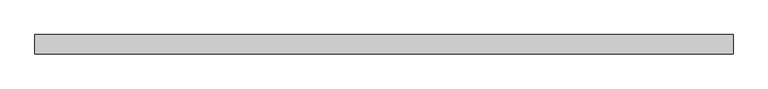
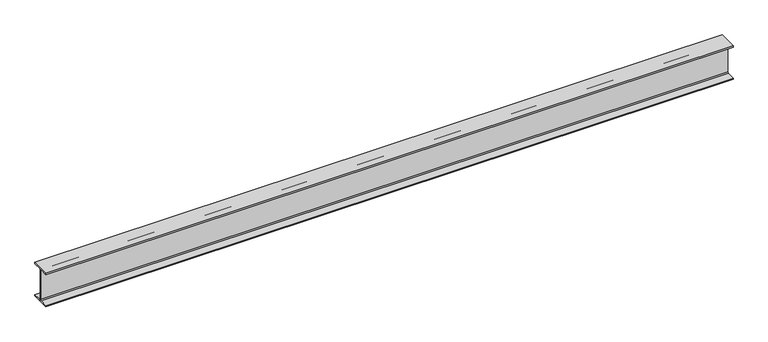
"""IFC4 building model written with IfcOpenShell, lengths in millimetres: beam geometry, Old_Steel Beam_H-KSD3502 : H_SB_ASB_H-350×175x7x11."""

import ifcopenshell
import ifcopenshell.guid

model = None  # the IFC model being written
_history = None  # IfcOwnerHistory: only IFC2X3 demands one
_inside = {}  # id of a spatial element -> (the spatial element, [elements in it])
_under = {}  # id of a project, library or spatial element -> (it, [spatial elements below it])
_declared = {}  # id of a project -> (the project, [libraries it declares])
_typed = {}  # id of a type object -> (the type object, [elements of that type])
_made_of = {}  # id of a material, layer set ... -> (it, [elements and type objects made of it])


def new_model(schema):
    """Start an empty IFC model of exactly this schema.

    Asked for "IFC4X3", IfcOpenShell would pick the latest addendum, in which some entities
    have other attributes; the version numbers below select the first issue.
    IFC2X3 requires an IfcOwnerHistory on every rooted entity: one is made here for all.
    """
    global model, _history
    if schema == "IFC4X3":
        model = ifcopenshell.file(schema_version=(4, 3, 0, 0))
    else:
        model = ifcopenshell.file(schema=schema)
    _inside.clear()
    _under.clear()
    _declared.clear()
    _typed.clear()
    _made_of.clear()
    _history = None
    if model.schema == "IFC2X3":
        org = make("IfcOrganization", Name="unknown")
        user = make(
            "IfcPersonAndOrganization",
            ThePerson=make("IfcPerson", FamilyName="unknown"),
            TheOrganization=org,
        )
        app = make(
            "IfcApplication",
            ApplicationDeveloper=org,
            Version="unknown",
            ApplicationFullName="unknown",
            ApplicationIdentifier="unknown",
        )
        _history = make(
            "IfcOwnerHistory",
            OwningUser=user,
            OwningApplication=app,
            ChangeAction="ADDED",
            CreationDate=0,
        )
    return model


def make(cls, **values):
    """One entity of the class cls with the attributes given. An attribute that is None is left unset."""
    return model.create_entity(
        cls, **{name: value for name, value in values.items() if value is not None}
    )


def rooted(cls, **values):
    """An entity with a GlobalId (a new one), such as an element, a storey or a relation."""
    return make(cls, GlobalId=ifcopenshell.guid.new(), OwnerHistory=_history, **values)


def si_unit(unit_type, name, prefix=None):
    """IfcSIUnit, for example si_unit("LENGTHUNIT", "METRE", prefix="MILLI")."""
    return make("IfcSIUnit", UnitType=unit_type, Prefix=prefix, Name=name)


def assignment(units):
    """IfcUnitAssignment: the units of a project."""
    return None if units is None else make("IfcUnitAssignment", Units=units)


def point(xyz):
    """IfcCartesianPoint."""
    return None if xyz is None else make("IfcCartesianPoint", Coordinates=xyz)


def direction(xyz):
    """IfcDirection."""
    return None if xyz is None else make("IfcDirection", DirectionRatios=xyz)


def frame(location, z_axis=None, x_axis=None):
    """IfcAxis2Placement3D, a coordinate frame: its origin and axes. An axis left out is left unset."""
    return make(
        "IfcAxis2Placement3D",
        Location=point(location),
        Axis=direction(z_axis),
        RefDirection=direction(x_axis),
    )


def frame_2d(location, x_axis=None):
    """IfcAxis2Placement2D, a coordinate frame in the plane: its origin and x axis."""
    return make(
        "IfcAxis2Placement2D", Location=point(location), RefDirection=direction(x_axis)
    )


def origin():
    """The frame at (0, 0, 0) with its axes left unset."""
    return frame((0.0, 0.0, 0.0))


def place(relative_to, where):
    """IfcLocalPlacement: puts the frame where relative to a parent placement (None: the world)."""
    return make(
        "IfcLocalPlacement", PlacementRelTo=relative_to, RelativePlacement=where
    )


def context(
    kind, dimensions, precision=None, world=None, true_north=None, identifier=None
):
    """IfcGeometricRepresentationContext, for example the 3D "Model" context."""
    return make(
        "IfcGeometricRepresentationContext",
        ContextIdentifier=identifier,
        ContextType=kind,
        CoordinateSpaceDimension=dimensions,
        Precision=precision,
        WorldCoordinateSystem=world,
        TrueNorth=true_north,
    )


def project(units=None, contexts=None):
    """IfcProject with its units and contexts."""
    return rooted(
        "IfcProject",
        Name="project",
        RepresentationContexts=contexts,
        UnitsInContext=assignment(units),
    )


def spatial(cls, under=None, at=None, **own):
    """A site, building, storey or space (cls), placed at a placement, below another one or the project."""
    s = rooted(cls, ObjectPlacement=at, **own)
    if under is not None:
        _under.setdefault(under.id(), (under, []))[1].append(s)
    return s


def polyline(points):
    """IfcPolyline through the points."""
    return make("IfcPolyline", Points=[point(p) for p in points])


def circle_curve(where, radius):
    """IfcCircle in the frame where."""
    return make("IfcCircle", Position=where, Radius=radius)


def trimmed(basis, trim1, trim2, sense, master):
    """IfcTrimmedCurve: the piece of a basis curve between two trims."""
    return make(
        "IfcTrimmedCurve",
        BasisCurve=basis,
        Trim1=trim1,
        Trim2=trim2,
        SenseAgreement=sense,
        MasterRepresentation=master,
    )


def segment(curve, same_sense, transition):
    """IfcCompositeCurveSegment."""
    return make(
        "IfcCompositeCurveSegment",
        Transition=transition,
        SameSense=same_sense,
        ParentCurve=curve,
    )


def composite_curve(segments, self_intersect=None):
    """IfcCompositeCurve: segments joined end to end."""
    return make("IfcCompositeCurve", Segments=segments, SelfIntersect=self_intersect)


def outline(outer, holes=None, kind="AREA"):
    """IfcArbitraryClosedProfileDef: a profile drawn as a closed curve; with holes, ...WithVoids."""
    if holes is None:
        return make("IfcArbitraryClosedProfileDef", ProfileType=kind, OuterCurve=outer)
    return make(
        "IfcArbitraryProfileDefWithVoids",
        ProfileType=kind,
        OuterCurve=outer,
        InnerCurves=holes,
    )


def extrude(swept, where, along, depth):
    """IfcExtrudedAreaSolid: the profile swept, set in the frame where, extruded along a direction by depth."""
    return make(
        "IfcExtrudedAreaSolid",
        SweptArea=swept,
        Position=where,
        ExtrudedDirection=direction(along),
        Depth=depth,
    )


def shape(context_of_items, identifier, shape_type, items):
    """IfcShapeRepresentation: the items that make up one representation, for example the "Body"."""
    return make(
        "IfcShapeRepresentation",
        ContextOfItems=context_of_items,
        RepresentationIdentifier=identifier,
        RepresentationType=shape_type,
        Items=items,
    )


def source(mapping_origin, context_of_items, identifier, shape_type, items):
    """IfcRepresentationMap: a shape defined once, which mapped items show again and again."""
    return make(
        "IfcRepresentationMap",
        MappingOrigin=mapping_origin,
        MappedRepresentation=shape(context_of_items, identifier, shape_type, items),
    )


def transform(
    local_origin,
    x_axis=None,
    y_axis=None,
    z_axis=None,
    scale=None,
    scale2=None,
    scale3=None,
    uniform=True,
):
    """IfcCartesianTransformationOperator3D, or its non-uniform kind. x_axis, y_axis, z_axis: its Axis1, 2, 3."""
    if uniform:
        return make(
            "IfcCartesianTransformationOperator3D",
            Axis1=direction(x_axis),
            Axis2=direction(y_axis),
            LocalOrigin=point(local_origin),
            Scale=scale,
            Axis3=direction(z_axis),
        )
    return make(
        "IfcCartesianTransformationOperator3DnonUniform",
        Axis1=direction(x_axis),
        Axis2=direction(y_axis),
        LocalOrigin=point(local_origin),
        Scale=scale,
        Axis3=direction(z_axis),
        Scale2=scale2,
        Scale3=scale3,
    )


def mapped(mapping_source, mapping_target):
    """IfcMappedItem: shows the shape of a source again, moved by a transform."""
    return make(
        "IfcMappedItem", MappingSource=mapping_source, MappingTarget=mapping_target
    )


def made_of(thing, what):
    """Note that an element or type object is made of a material, layer set ...; save() writes the relation."""
    if what is not None:
        _made_of.setdefault(what.id(), (what, []))[1].append(thing)
    return thing


def element(
    cls,
    number,
    at=None,
    inside=None,
    cuts=None,
    type_object=None,
    material=None,
    context=None,
    identifier="Body",
    shape_type=None,
    held_by="IfcProductDefinitionShape",
    body=None,
    shapes=None,
    **own,
):
    """One element of the class cls, such as IfcWall. Its Tag is "e" and its number.

    at: its placement. inside: the storey or other place that contains it. cuts: it is an
    opening in that element (IfcRelVoidsElement). A single representation is given by context,
    identifier, shape_type and body (its items); several are given by shapes. held_by: the class
    of the entity that holds the representations. save() writes the other relations.
    """
    e = rooted(cls, Tag="e%d" % number, ObjectPlacement=at, **own)
    if body is not None:
        shapes = [shape(context, identifier, shape_type, body)]
    if shapes is not None:
        e.Representation = make(held_by, Representations=shapes)
    if inside is not None:
        _inside.setdefault(inside.id(), (inside, []))[1].append(e)
    if cuts is not None:
        rooted(
            "IfcRelVoidsElement", RelatingBuildingElement=cuts, RelatedOpeningElement=e
        )
    if type_object is not None:
        _typed.setdefault(type_object.id(), (type_object, []))[1].append(e)
    return made_of(e, material)


def aggregate(whole, parts):
    """IfcRelAggregates: a whole, such as a stair, and the parts it consists of."""
    return rooted("IfcRelAggregates", RelatingObject=whole, RelatedObjects=parts)


def save(model, path):
    """Write the relations noted so far, then the file.

    IfcRelAggregates (storeys below a building ...), IfcRelContainedInSpatialStructure (elements
    in a storey), IfcRelDefinesByType, IfcRelAssociatesMaterial and IfcRelDeclares: one each for
    every whole, place, type object, material and project.
    """
    for whole, parts in _under.values():
        aggregate(whole, parts)
    for where, things in _inside.values():
        rooted(
            "IfcRelContainedInSpatialStructure",
            RelatedElements=things,
            RelatingStructure=where,
        )
    for kind, things in _typed.values():
        rooted("IfcRelDefinesByType", RelatedObjects=things, RelatingType=kind)
    for what, things in _made_of.values():
        rooted("IfcRelAssociatesMaterial", RelatedObjects=things, RelatingMaterial=what)
    for by, libraries in _declared.values():
        rooted("IfcRelDeclares", RelatingContext=by, RelatedDefinitions=libraries)
    model.write(path)


def beam_8e561ac9(model_context):
    return source(origin(), model_context, "Body", "SweptSolid", [
        extrude(outline(composite_curve([segment(polyline([(82.5, -141.5), (82.5, -151.7), (-82.5, -151.7), (-82.5, -141.5), (-11.9, -141.5)]), True, "CONTINUOUS"), segment(trimmed(circle_curve(frame_2d((-11.9, -132.6)), 8.9), [point((-11.9, -141.5))], [point((-3.0, -132.6))], True, "CARTESIAN"), True, "CONTINUOUS"), segment(polyline([(-3.0, -132.6), (-3.0, 132.6)]), True, "CONTINUOUS"), segment(trimmed(circle_curve(frame_2d((-11.9, 132.6)), 8.9), [point((-3.0, 132.6))], [point((-11.9, 141.5))], True, "CARTESIAN"), True, "CONTINUOUS"), segment(polyline([(-11.9, 141.5), (-82.5, 141.5), (-82.5, 151.7), (82.5, 151.7), (82.5, 141.5), (11.9, 141.5)]), True, "CONTINUOUS"), segment(trimmed(circle_curve(frame_2d((11.9, 132.6)), 8.9), [point((11.9, 141.5))], [point((3.0, 132.6))], True, "CARTESIAN"), True, "CONTINUOUS"), segment(polyline([(3.0, 132.6), (3.0, -132.6)]), True, "CONTINUOUS"), segment(trimmed(circle_curve(frame_2d((11.9, -132.6)), 8.9), [point((3.0, -132.6))], [point((11.9, -141.5))], True, "CARTESIAN"), True, "CONTINUOUS"), segment(polyline([(11.9, -141.5), (82.5, -141.5)]), True, "CONTINUOUS")], self_intersect=False)), frame((-2898.0675435, 0.0, 0.0), z_axis=(1.0, 0.0, 0.0), x_axis=(0.0, 1.0, 0.0)), (0.0, 0.0, 1.0), 5918.7701357),
    ])


if __name__ == "__main__":
    model = new_model("IFC4")
    model_context = context("Model", 3, world=origin())
    ifc_project = project(units=[si_unit("LENGTHUNIT", "METRE", prefix="MILLI")], contexts=[model_context])
    site = spatial("IfcSite", under=ifc_project)
    building = spatial("IfcBuilding", under=site)
    placement = place(None, origin())
    beam_shape = beam_8e561ac9(model_context)
    element("IfcBeam", 1, ObjectType="Old_Steel Beam_H-KSD3502 : H_SB_ASB_H-350×175x7x11", at=placement, inside=building, context=model_context, shape_type="MappedRepresentation", body=[
        mapped(beam_shape, transform((0.0, 0.0, 0.0), x_axis=(1.0, 0.0, 0.0), y_axis=(0.0, 1.0, 0.0), z_axis=(0.0, 0.0, 1.0))),
    ])
    save(model, "model.ifc")

# Revit data of these elements
# Type "Old_Steel Beam_H-KSD3502 : H_SB_ASB_H-350×175x7x11"
#   Width = 17.5 cm
#   Web Thickness = 0.7 cm
#   Web Fillet = 1.4 cm
#   Warping Constant = 282290.0 cm⁶
#   Torsional Moment of Inertia = 19.4042 cm⁴
#   Torsional Modulus = 1.0 cm³
#   Section Area = 63.14 cm²
#   Plastic Modulus weak axis = 174.0 cm³
#   Plastic Modulus strong axis = 868.0 cm³
#   Perimeter = 1.36 m²/m
#   Nominal Weight = 49.60 kgf/m
#   Moment of Inertia weak axis = 984.00 cm⁴
#   Moment of Inertia strong axis = 13600.00 cm⁴
#   Height = 35.0 cm
#   Flange Thickness = 1.1 cm
#   Elastic Modulus weak axis = 112.0 cm³
#   Elastic Modulus strong axis = 775.0 cm³
#   Centroid Vertical = 17.5 cm
#   Centroid Horizontal = 8.75 cm
#   Length [instance default] = 1.5240 m
#   Structural Material [instance default] = Steel, 45-345
#   Assembly Code = ""
# Element 1 (IfcBeam, "Old_Steel Beam_H-KSD3502 : H_SB_ASB_H-350×175x7x11")
#   Structural Material = none
# Materials
#   "Steel, 45-345": class "Metal", colour RGB 189 187 185, transparency 0, Description = "Steel 345 MPa", Cost = 0
